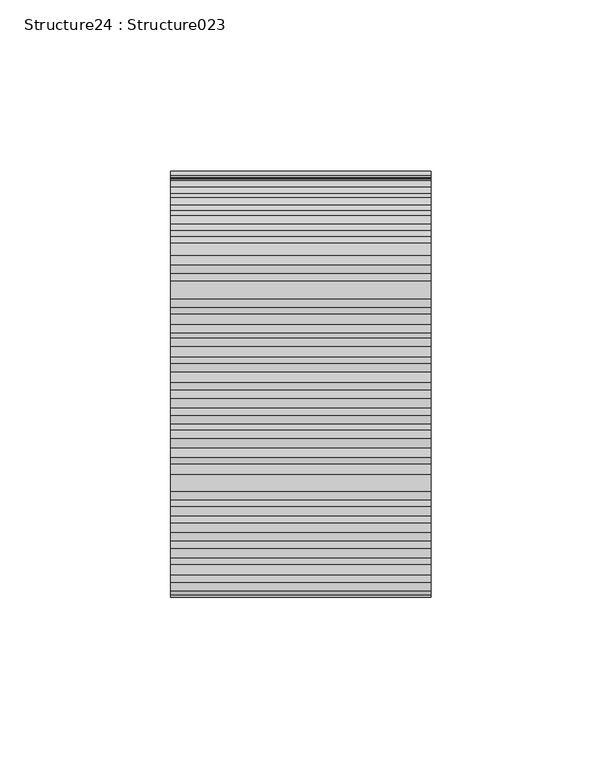
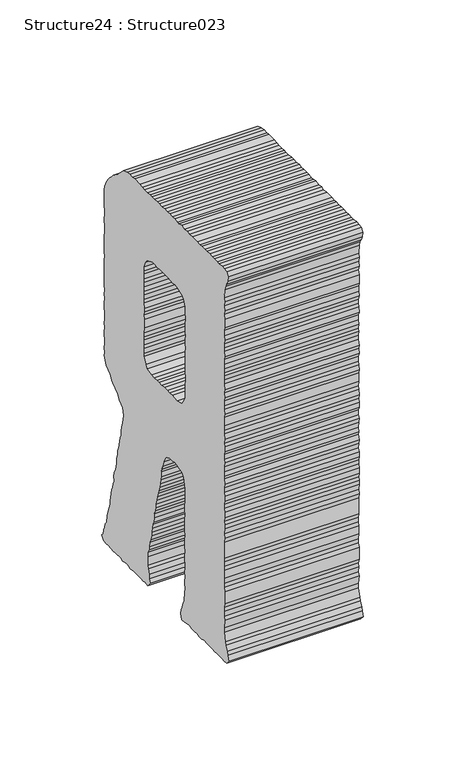
"""IFC4 building model written with IfcOpenShell, lengths in millimetres: proxy geometry, Structure24 : Structure023."""

from ifc_helpers import new_model, si_unit, frame, origin, place, context, project, spatial, polyline, outline, extrude, source, transform, mapped, element, save


def structure24_structure023_ec477ba6(model_context):
    return source(origin(), model_context, "Body", "SweptSolid", [
        extrude(outline(polyline([(1.8740926, 0.0), (4.6350237, -0.4605769), (6.8121729, -0.5076971), (9.8126052, -1.3242981), (11.9468116, -1.6803252), (14.0311121, -2.3406622), (17.1848842, -2.2380669), (18.9694706, -2.8518412), (24.156244, -3.7170958), (26.9450766, -3.8662567), (29.3338255, -4.580817), (31.4780595, -4.9385169), (33.8656948, -5.649456), (36.7194746, -5.4968162), (39.3649949, -6.5668461), (41.5415866, -6.6173088), (44.3546525, -6.7705122), (48.5143396, -8.0931346), (51.5652354, -8.6020833), (53.8031537, -8.3467058), (56.4386465, -9.4150629), (58.6899349, -9.1619159), (61.4283039, -9.6187291), (63.157135, -10.5358374), (65.5971832, -10.9428848), (68.7501196, -10.8401502), (71.0964833, -11.8602749), (73.333566, -11.6047581), (77.5517934, -14.5020391), (78.4231709, -16.8470127), (79.9915604, -18.6744024), (82.1900172, -20.6068996), (83.6521879, -23.0452757), (84.3173968, -24.7262919), (85.7836063, -27.1662005), (87.9265857, -29.4055136), (89.4941388, -31.2379172), (90.4683934, -32.9661937), (94.2367722, -34.8479494), (99.3227596, -34.4432741), (102.465807, -34.3431842), (104.7031679, -34.0911494), (107.454907, -34.550193), (109.7434282, -33.9863277), (111.9813466, -33.7309503), (114.7838273, -33.8858234), (117.0582814, -33.3239059), (119.3087335, -33.0757727), (121.7943707, -33.1734958), (124.3441188, -32.9744321), (127.3858225, -33.4818474), (131.8743332, -32.972348), (134.5120556, -32.1583956), (137.3574791, -32.0043619), (140.0526265, -32.7717532), (142.0282021, -32.1634124), (144.8312404, -32.3149431), (146.8671684, -31.3963053), (149.6597601, -31.5538233), (151.9060348, -31.2998399), (154.7464445, -31.1449697), (156.8814865, -31.5011362), (159.4362493, -31.2977558), (162.3778632, -30.5362161), (165.2185516, -30.3796747), (169.9539439, -30.2334428), (171.9933532, -29.3196801), (174.5302887, -29.1150436), (176.5189564, -28.5054512), (179.3680004, -28.3554571), (181.0954405, -27.3862163), (183.2240748, -29.6239953), (183.1306685, -32.1146471), (182.5116023, -33.894915), (182.4174991, -36.389745), (181.9599889, -39.1322922), (181.2388821, -41.5242435), (180.4749712, -46.1035118), (180.7355018, -48.341431), (179.609856, -51.2894496), (179.3049886, -53.1169788), (179.5139413, -55.6640821), (178.7024942, -58.6593619), (177.5311177, -65.6811852), (177.4781465, -67.8676651), (176.5044465, -69.9048438), (176.7149326, -72.4427552), (173.2565712, -74.3763615), (171.2734749, -73.1093551), (168.885701, -72.3940985), (166.2351669, -71.3232323), (164.5063358, -70.4061241), (159.6320891, -69.593005), (156.8803499, -69.1339614), (154.5412265, -70.0011615), (152.3547459, -69.9533435), (149.5664718, -69.795687), (147.2131426, -70.6605172), (144.3724541, -70.8170586), (141.8833366, -70.7093071), (139.3844686, -70.608518), (136.8986928, -70.5064774), (134.5467569, -71.3681045), (131.7579251, -71.2137904), (129.2671348, -71.1160665), (126.6660875, -71.6226432), (124.443072, -71.8762122), (122.2938241, -71.5176759), (119.453275, -71.6733816), (116.9128576, -71.8782963), (114.3125073, -72.3806947), (112.3869755, -72.6941965), (109.4831512, -73.1468284), (107.2968108, -73.0930216), (104.4479054, -73.2473333), (102.209987, -73.5027107), (99.1549131, -72.993065), (97.2309146, -73.2973749), (94.629031, -73.8089652), (91.4760946, -73.9116999), (87.1480256, -75.3850102), (85.0193882, -78.7901217), (84.5104395, -81.8410174), (83.6023846, -83.5670643), (83.6959265, -86.7236205), (84.2026424, -91.1979246), (85.779527, -93.0310259), (89.2951739, -94.5536915), (91.9312235, -95.6238592), (98.9446905, -96.7938418), (101.4954144, -96.5889287), (104.5463101, -97.0978773), (106.8832031, -98.1181399), (109.3815134, -98.2222716), (111.2556067, -98.2171184), (113.6390631, -98.9325136), (116.7033289, -99.4436927), (118.7792731, -100.1026355), (121.6291536, -99.9476276), (124.0817362, -100.356766), (125.8526736, -100.9699812), (128.2495009, -101.6824536), (131.4035517, -101.5781871), (133.8419286, -101.9849558), (135.8754868, -102.9546162), (138.0105289, -103.3107827), (140.8604093, -103.1557747), (143.500637, -104.2266394), (145.9864128, -104.3286801), (147.8222983, -104.6349415), (150.5191178, -105.3974584), (152.7472874, -105.138737), (158.3486281, -105.4444439), (160.3364595, -104.8398653), (163.4903709, -104.7364346), (165.5162706, -103.8212771), (168.3701898, -103.6678018), (171.2168648, -105.4009526), (170.404442, -108.4020819), (169.3851545, -110.7382786), (169.0281516, -112.8783345), (168.9710021, -115.0641173), (168.8269938, -117.8581039), (168.1058869, -120.2500552), (168.0629434, -122.4382077), (167.6553384, -124.8815984), (166.68735, -126.9102822), (166.5787621, -129.4044137), (165.7137863, -134.5895158), (165.6201012, -137.0818389), (164.9505723, -139.1646059), (164.0847601, -144.3547219), (164.042653, -146.5378608), (163.6863471, -148.6737385), (160.5817832, -150.3554478), (157.9819899, -148.9855644), (155.9583205, -148.0132592), (153.4133075, -146.3407379), (151.679602, -145.4219577), (147.0005227, -143.3874206), (144.5613102, -142.9805126), (139.5730459, -142.7736432), (137.5528571, -141.8113664), (134.4470424, -141.6007379), (132.3527135, -140.9438814), (129.812018, -141.1453141), (122.7893591, -139.9737981), (120.4566434, -138.9593857), (118.017431, -138.5524777), (114.9024244, -138.3403158), (110.34154, -137.5794717), (107.9438763, -136.872013), (105.508842, -136.465802), (103.0197245, -136.3580506), (93.5628669, -134.7804629), (91.0720765, -134.682739), (88.6760856, -133.9652529), (85.5685981, -133.7646519), (83.1343995, -133.3585803), (81.3492563, -132.7429954), (78.8634798, -132.6461079), (75.7983782, -132.1347894), (73.4107437, -131.4186972), (71.2890718, -131.0647611), (69.0890816, -131.0155483), (66.3507126, -130.5587352), (64.3079617, -129.5926946), (61.5146736, -129.4342016), (59.0288971, -129.3373141), (56.3920111, -128.2721602), (54.4970285, -128.263522), (52.1077212, -127.5574574), (49.0069204, -127.3476653), (46.5169656, -127.2500808), (44.7859057, -126.3360363), (41.7308318, -125.8263906), (39.8059977, -126.1305609), (37.0450666, -125.669984), (34.9749726, -125.0068637), (32.4850179, -124.9092792), (29.4714943, -124.0887766), (27.698884, -123.485589), (24.9106099, -123.3279325), (19.7104663, -122.4604475), (17.8280166, -122.4642066), (15.1403899, -121.6980699), (13.0560886, -121.0428862), (10.3026782, -120.5835639), (8.0669887, -120.8358775), (5.379362, -120.0697408), (3.1802075, -120.0206674), (0.2391511, -118.904772), (-2.2092533, -118.4963306), (-4.6933571, -118.3894155), (-6.4668029, -117.7860885), (-8.968455, -117.6762461), (-11.3535842, -116.9708785), (-14.4053156, -116.4617904), (-16.3426841, -116.7638697), (-19.3420019, -115.9457369), (-21.1288179, -115.3401795), (-23.5621809, -114.9342473), (-26.103712, -115.1355406), (-28.499703, -114.4180544), (-31.5505987, -113.9091057), (-33.438062, -113.9120285), (-38.3114731, -113.0990488), (-40.9617292, -112.0316645), (-43.4982466, -112.2337942), (-46.1850377, -111.4677969), (-48.6900339, -111.3677032), (-50.773498, -110.7023526), (-56.0617552, -110.4505919), (-58.6030084, -110.6553671), (-60.6381, -111.5689912), (-63.2309311, -112.0829506), (-66.0289548, -111.9271031), (-68.277456, -110.2945982), (-68.1688682, -107.8004668), (-67.8133987, -105.6696029), (-67.0047358, -102.6652698), (-66.699729, -100.8369049), (-66.5398421, -98.0352606), (-65.885216, -95.9543018), (-65.7776039, -93.4660199), (-65.3193968, -90.7192946), (-64.6632373, -88.6291438), (-64.5046049, -85.8350202), (-63.9000233, -84.0540536), (-63.7922719, -81.5649361), (-62.9770618, -76.6781548), (-62.1696535, -73.6813424), (-62.4674161, -71.7489884), (-61.405882, -69.1029097), (-61.5515594, -66.2588802), (-60.839784, -63.8662312), (-60.235063, -62.084429), (-60.4306456, -59.5395561), (-59.7703087, -57.4552555), (-59.6169689, -54.6619668), (-58.9060299, -52.2743315), (-58.8531974, -50.0835341), (-57.7416187, -47.1374632), (-57.6330308, -44.6433317), (-57.3274665, -42.8116245), (-56.5185248, -39.8056201), (-56.1125925, -37.372257), (-56.1559505, -35.7889656), (-55.4507222, -33.404672), (-54.9409372, -30.3487624), (-54.9353658, -28.4721638), (-54.8317917, -25.977196), (-53.9665372, -20.7904226), (-53.3063396, -18.7069577), (-53.2027656, -16.2119898), (-52.1419284, -13.5700893), (-50.299217, -10.1181388), (-47.8700306, -8.6389751), (-46.0320541, -7.0586095), (-43.5782169, -5.5861347), (-41.6529647, -3.4053649), (-40.177142, -2.0755022), (-38.1014758, -0.8568707), (-35.8985598, 0.9752511), (-34.1867194, 1.9385053), (-31.4327507, 3.3617712), (-27.1605763, 4.5309119), (-24.9747927, 4.4789158), (-20.0871758, 3.6635663), (-16.9941729, 3.463664), (-15.1482599, 3.1557298), (-12.8119237, 2.1372778), (-10.3768894, 1.7310668), (-7.8356363, 1.9358421), (-2.4383768, 0.4067686), (0.0, 0.0), (1.8740926, 0.0)]), holes=[polyline([(45.4437656, -75.3239371), (46.2660765, -72.3253162), (46.2574422, -70.4463478), (46.7672273, -67.3904382), (47.8422702, -64.7509075), (47.9458442, -62.2559397), (48.2514086, -60.4242324), (49.0653641, -57.4190644), (48.8038585, -55.1818415), (48.9787869, -50.5086138), (46.9823212, -49.2342239), (43.982586, -46.5393522), (41.7977774, -46.4866598), (38.7468817, -45.9777111), (36.9607626, -45.3679756), (34.2132016, -44.909629), (32.0359138, -44.8581913), (29.6025508, -44.4522591), (26.4858713, -44.2501248), (21.6074465, -43.4363087), (19.2114556, -42.7188225), (17.024, -42.6717008), (14.8889579, -42.3155343), (12.2527689, -41.2462021), (10.1177268, -40.8900356), (7.3153856, -40.7343268), (5.1795079, -40.3780209), (2.7950757, -39.6684751), (-0.0072656, -39.5127663), (-2.0917056, -38.853265), (-4.8434447, -38.3942215), (-7.0299245, -38.3412503), (-9.1009944, -37.6839795), (-13.0235494, -38.6005263), (-15.1648599, -40.1251367), (-17.7596418, -44.3938268), (-18.1673862, -46.838053), (-17.8604309, -48.7667872), (-18.8797192, -51.1081371), (-20.1527182, -58.7391369), (-20.3609777, -61.835899), (-20.3547116, -63.7187668), (-21.3731636, -66.055103), (-21.1692247, -68.6013699), (-20.3581997, -73.1307331), (-19.4353829, -75.1622049), (-15.9786951, -76.9919645), (-13.8444887, -77.3479916), (-8.4466723, -78.8788756), (-6.2185028, -78.6201542), (-1.032565, -79.4852694), (0.6976585, -80.4043277), (3.5001392, -80.559201), (5.6867593, -80.6061833), (8.6269792, -81.7270925), (10.5085924, -81.7283471), (19.9704638, -83.3067711), (22.7687671, -83.4557941), (24.8023253, -84.4254545), (27.2540722, -84.8344535), (30.0440185, -84.9872358), (32.2314741, -85.0343575), (34.6790428, -85.4426595), (37.6691688, -86.2592591), (40.9758623, -85.2399745), (43.3792361, -84.0751521), (45.3488258, -79.6978733), (45.4437656, -75.3239371)])]), frame((-35624.0862846, 275666.2565233, 4168.7393153), z_axis=(1.0, 0.0, 1.354250045437766e-12), x_axis=(1.3388890846442404e-12, 0.16454559576290828, -0.9863694778910334)), (0.0, 0.0, 1.0), 76.2),
    ])


if __name__ == "__main__":
    model = new_model("IFC4")
    model_context = context("Model", 3, world=origin())
    ifc_project = project(units=[si_unit("LENGTHUNIT", "METRE", prefix="MILLI")], contexts=[model_context])
    site = spatial("IfcSite", under=ifc_project)
    building = spatial("IfcBuilding", under=site)
    placement = place(None, origin())
    structure24_structure023_shape = structure24_structure023_ec477ba6(model_context)
    element("IfcBuildingElementProxy", 1, Name="Structure24 : Structure023", ObjectType="Structure24 : Structure023", at=placement, inside=building, context=model_context, shape_type="MappedRepresentation", body=[
        mapped(structure24_structure023_shape, transform((0.0, 0.0, 0.0), x_axis=(1.0, 0.0, 0.0), y_axis=(0.0, 1.0, 0.0), z_axis=(0.0, 0.0, 1.0))),
    ])
    save(model, "model.ifc")

# Revit data of these elements
# Type "Structure24 : Structure023"
#   NameOverride = "Structure023"
# Element 1 (IfcBuildingElementProxy, "Structure24 : Structure023")
#   Materials on its faces: "BRUSHED ALUMINUM LETTERING"
# Materials
#   "BRUSHED ALUMINUM LETTERING": class "Unassigned", colour RGB 169 181 186, transparency 0, Cost = 0
